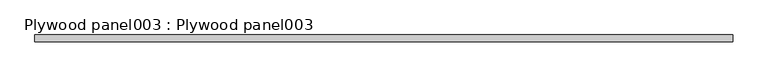
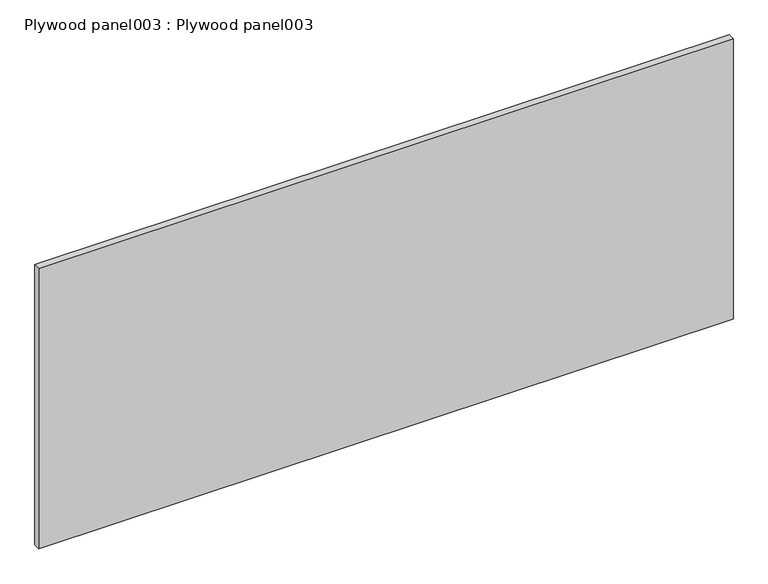
"""IFC4 building model written with IfcOpenShell, lengths in millimetres: proxy geometry, Plywood panel003 : Plywood panel003."""

from ifc_helpers import new_model, si_unit, frame, origin, place, context, project, spatial, polyline, outline, extrude, source, transform, mapped, element, save


def plywood_panel003_plywood_panel003_feb83b17(model_context):
    return source(origin(), model_context, "Body", "SweptSolid", [
        extrude(outline(polyline([(14383.0178845, -4389.8932763), (14383.0178845, -4408.9401513), (12383.0178845, -4408.9401513), (12383.0178845, -4389.8932763), (14383.0178845, -4389.8932763)])), frame((0.0, 0.0, 40201.5164062), z_axis=(0.0, 0.0, 1.0), x_axis=(1.0, 0.0, 0.0)), (0.0, 0.0, 1.0), 854.1631875),
    ])


if __name__ == "__main__":
    model = new_model("IFC4")
    model_context = context("Model", 3, world=origin())
    ifc_project = project(units=[si_unit("LENGTHUNIT", "METRE", prefix="MILLI")], contexts=[model_context])
    site = spatial("IfcSite", under=ifc_project)
    building = spatial("IfcBuilding", under=site)
    placement = place(None, origin())
    plywood_panel003_plywood_panel003_shape = plywood_panel003_plywood_panel003_feb83b17(model_context)
    element("IfcBuildingElementProxy", 1, Name="Plywood panel003 : Plywood panel003", ObjectType="Plywood panel003 : Plywood panel003", at=placement, inside=building, context=model_context, shape_type="MappedRepresentation", body=[
        mapped(plywood_panel003_plywood_panel003_shape, transform((0.0, 0.0, 0.0), x_axis=(1.0, 0.0, 0.0), y_axis=(0.0, 1.0, 0.0), z_axis=(0.0, 0.0, 1.0))),
    ])
    save(model, "model.ifc")

# Revit data of these elements
# Type "Plywood panel003 : Plywood panel003"
#   NameOverride = "Plywood panel003"
# Element 1 (IfcBuildingElementProxy, "Plywood panel003 : Plywood panel003")
#   Materials on its faces: "CDX PLYWOOD - SEE STRUCTURAL DWGS"
# Materials
#   "CDX PLYWOOD - SEE STRUCTURAL DWGS": class "Unassigned", colour RGB 177 130 114, transparency 0, Cost = 0
